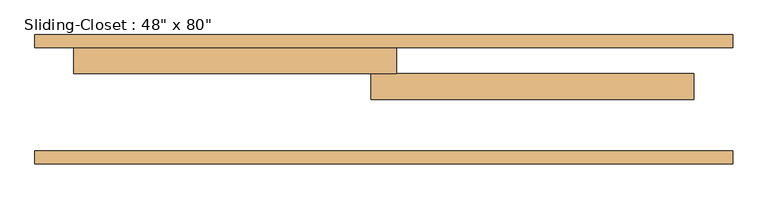
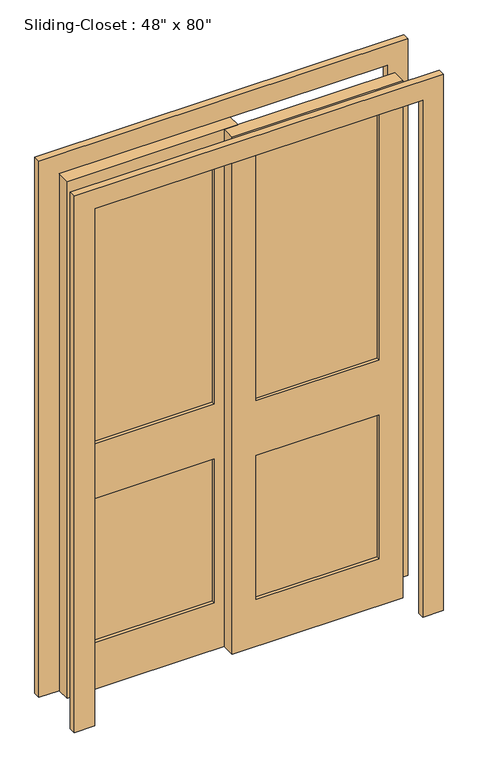
"""IFC4 building model written with IfcOpenShell, lengths in millimetres: door geometry."""

import ifcopenshell
import ifcopenshell.guid

model = None  # the IFC model being written
_history = None  # IfcOwnerHistory: only IFC2X3 demands one
_inside = {}  # id of a spatial element -> (the spatial element, [elements in it])
_under = {}  # id of a project, library or spatial element -> (it, [spatial elements below it])
_declared = {}  # id of a project -> (the project, [libraries it declares])
_typed = {}  # id of a type object -> (the type object, [elements of that type])
_made_of = {}  # id of a material, layer set ... -> (it, [elements and type objects made of it])


def new_model(schema):
    """Start an empty IFC model of exactly this schema.

    Asked for "IFC4X3", IfcOpenShell would pick the latest addendum, in which some entities
    have other attributes; the version numbers below select the first issue.
    IFC2X3 requires an IfcOwnerHistory on every rooted entity: one is made here for all.
    """
    global model, _history
    if schema == "IFC4X3":
        model = ifcopenshell.file(schema_version=(4, 3, 0, 0))
    else:
        model = ifcopenshell.file(schema=schema)
    _inside.clear()
    _under.clear()
    _declared.clear()
    _typed.clear()
    _made_of.clear()
    _history = None
    if model.schema == "IFC2X3":
        org = make("IfcOrganization", Name="unknown")
        user = make(
            "IfcPersonAndOrganization",
            ThePerson=make("IfcPerson", FamilyName="unknown"),
            TheOrganization=org,
        )
        app = make(
            "IfcApplication",
            ApplicationDeveloper=org,
            Version="unknown",
            ApplicationFullName="unknown",
            ApplicationIdentifier="unknown",
        )
        _history = make(
            "IfcOwnerHistory",
            OwningUser=user,
            OwningApplication=app,
            ChangeAction="ADDED",
            CreationDate=0,
        )
    return model


def make(cls, **values):
    """One entity of the class cls with the attributes given. An attribute that is None is left unset."""
    return model.create_entity(
        cls, **{name: value for name, value in values.items() if value is not None}
    )


def rooted(cls, **values):
    """An entity with a GlobalId (a new one), such as an element, a storey or a relation."""
    return make(cls, GlobalId=ifcopenshell.guid.new(), OwnerHistory=_history, **values)


def si_unit(unit_type, name, prefix=None):
    """IfcSIUnit, for example si_unit("LENGTHUNIT", "METRE", prefix="MILLI")."""
    return make("IfcSIUnit", UnitType=unit_type, Prefix=prefix, Name=name)


def assignment(units):
    """IfcUnitAssignment: the units of a project."""
    return None if units is None else make("IfcUnitAssignment", Units=units)


def point(xyz):
    """IfcCartesianPoint."""
    return None if xyz is None else make("IfcCartesianPoint", Coordinates=xyz)


def direction(xyz):
    """IfcDirection."""
    return None if xyz is None else make("IfcDirection", DirectionRatios=xyz)


def frame(location, z_axis=None, x_axis=None):
    """IfcAxis2Placement3D, a coordinate frame: its origin and axes. An axis left out is left unset."""
    return make(
        "IfcAxis2Placement3D",
        Location=point(location),
        Axis=direction(z_axis),
        RefDirection=direction(x_axis),
    )


def origin():
    """The frame at (0, 0, 0) with its axes left unset."""
    return frame((0.0, 0.0, 0.0))


def place(relative_to, where):
    """IfcLocalPlacement: puts the frame where relative to a parent placement (None: the world)."""
    return make(
        "IfcLocalPlacement", PlacementRelTo=relative_to, RelativePlacement=where
    )


def context(
    kind, dimensions, precision=None, world=None, true_north=None, identifier=None
):
    """IfcGeometricRepresentationContext, for example the 3D "Model" context."""
    return make(
        "IfcGeometricRepresentationContext",
        ContextIdentifier=identifier,
        ContextType=kind,
        CoordinateSpaceDimension=dimensions,
        Precision=precision,
        WorldCoordinateSystem=world,
        TrueNorth=true_north,
    )


def project(units=None, contexts=None):
    """IfcProject with its units and contexts."""
    return rooted(
        "IfcProject",
        Name="project",
        RepresentationContexts=contexts,
        UnitsInContext=assignment(units),
    )


def spatial(cls, under=None, at=None, **own):
    """A site, building, storey or space (cls), placed at a placement, below another one or the project."""
    s = rooted(cls, ObjectPlacement=at, **own)
    if under is not None:
        _under.setdefault(under.id(), (under, []))[1].append(s)
    return s


def polyline(points):
    """IfcPolyline through the points."""
    return make("IfcPolyline", Points=[point(p) for p in points])


def outline(outer, holes=None, kind="AREA"):
    """IfcArbitraryClosedProfileDef: a profile drawn as a closed curve; with holes, ...WithVoids."""
    if holes is None:
        return make("IfcArbitraryClosedProfileDef", ProfileType=kind, OuterCurve=outer)
    return make(
        "IfcArbitraryProfileDefWithVoids",
        ProfileType=kind,
        OuterCurve=outer,
        InnerCurves=holes,
    )


def extrude(swept, where, along, depth):
    """IfcExtrudedAreaSolid: the profile swept, set in the frame where, extruded along a direction by depth."""
    return make(
        "IfcExtrudedAreaSolid",
        SweptArea=swept,
        Position=where,
        ExtrudedDirection=direction(along),
        Depth=depth,
    )


def shape(context_of_items, identifier, shape_type, items):
    """IfcShapeRepresentation: the items that make up one representation, for example the "Body"."""
    return make(
        "IfcShapeRepresentation",
        ContextOfItems=context_of_items,
        RepresentationIdentifier=identifier,
        RepresentationType=shape_type,
        Items=items,
    )


def source(mapping_origin, context_of_items, identifier, shape_type, items):
    """IfcRepresentationMap: a shape defined once, which mapped items show again and again."""
    return make(
        "IfcRepresentationMap",
        MappingOrigin=mapping_origin,
        MappedRepresentation=shape(context_of_items, identifier, shape_type, items),
    )


def transform(
    local_origin,
    x_axis=None,
    y_axis=None,
    z_axis=None,
    scale=None,
    scale2=None,
    scale3=None,
    uniform=True,
):
    """IfcCartesianTransformationOperator3D, or its non-uniform kind. x_axis, y_axis, z_axis: its Axis1, 2, 3."""
    if uniform:
        return make(
            "IfcCartesianTransformationOperator3D",
            Axis1=direction(x_axis),
            Axis2=direction(y_axis),
            LocalOrigin=point(local_origin),
            Scale=scale,
            Axis3=direction(z_axis),
        )
    return make(
        "IfcCartesianTransformationOperator3DnonUniform",
        Axis1=direction(x_axis),
        Axis2=direction(y_axis),
        LocalOrigin=point(local_origin),
        Scale=scale,
        Axis3=direction(z_axis),
        Scale2=scale2,
        Scale3=scale3,
    )


def mapped(mapping_source, mapping_target):
    """IfcMappedItem: shows the shape of a source again, moved by a transform."""
    return make(
        "IfcMappedItem", MappingSource=mapping_source, MappingTarget=mapping_target
    )


def made_of(thing, what):
    """Note that an element or type object is made of a material, layer set ...; save() writes the relation."""
    if what is not None:
        _made_of.setdefault(what.id(), (what, []))[1].append(thing)
    return thing


def element(
    cls,
    number,
    at=None,
    inside=None,
    cuts=None,
    type_object=None,
    material=None,
    context=None,
    identifier="Body",
    shape_type=None,
    held_by="IfcProductDefinitionShape",
    body=None,
    shapes=None,
    **own,
):
    """One element of the class cls, such as IfcWall. Its Tag is "e" and its number.

    at: its placement. inside: the storey or other place that contains it. cuts: it is an
    opening in that element (IfcRelVoidsElement). A single representation is given by context,
    identifier, shape_type and body (its items); several are given by shapes. held_by: the class
    of the entity that holds the representations. save() writes the other relations.
    """
    e = rooted(cls, Tag="e%d" % number, ObjectPlacement=at, **own)
    if body is not None:
        shapes = [shape(context, identifier, shape_type, body)]
    if shapes is not None:
        e.Representation = make(held_by, Representations=shapes)
    if inside is not None:
        _inside.setdefault(inside.id(), (inside, []))[1].append(e)
    if cuts is not None:
        rooted(
            "IfcRelVoidsElement", RelatingBuildingElement=cuts, RelatedOpeningElement=e
        )
    if type_object is not None:
        _typed.setdefault(type_object.id(), (type_object, []))[1].append(e)
    return made_of(e, material)


def aggregate(whole, parts):
    """IfcRelAggregates: a whole, such as a stair, and the parts it consists of."""
    return rooted("IfcRelAggregates", RelatingObject=whole, RelatedObjects=parts)


def save(model, path):
    """Write the relations noted so far, then the file.

    IfcRelAggregates (storeys below a building ...), IfcRelContainedInSpatialStructure (elements
    in a storey), IfcRelDefinesByType, IfcRelAssociatesMaterial and IfcRelDeclares: one each for
    every whole, place, type object, material and project.
    """
    for whole, parts in _under.values():
        aggregate(whole, parts)
    for where, things in _inside.values():
        rooted(
            "IfcRelContainedInSpatialStructure",
            RelatedElements=things,
            RelatingStructure=where,
        )
    for kind, things in _typed.values():
        rooted("IfcRelDefinesByType", RelatedObjects=things, RelatingType=kind)
    for what, things in _made_of.values():
        rooted("IfcRelAssociatesMaterial", RelatedObjects=things, RelatingMaterial=what)
    for by, libraries in _declared.values():
        rooted("IfcRelDeclares", RelatingContext=by, RelatedDefinitions=libraries)
    model.write(path)


def door_5d877b8f(model_context):
    return source(origin(), model_context, "Body", "SweptSolid", [
        extrude(outline(polyline([(-63.5, 190.5), (-520.7, 190.5), (-520.7, 215.9), (-63.5, 215.9), (-63.5, 190.5)])), frame((0.0, 0.0, 965.2), z_axis=(0.0, 0.0, 1.0), x_axis=(1.0, 0.0, 0.0)), (0.0, 0.0, 1.0), 977.9),
        extrude(outline(polyline([(-63.5, 190.5), (-520.7, 190.5), (-520.7, 215.9), (-63.5, 215.9), (-63.5, 190.5)])), frame((0.0, 0.0, 184.15), z_axis=(0.0, 0.0, 1.0), x_axis=(1.0, 0.0, 0.0)), (0.0, 0.0, 1.0), 565.15),
        extrude(outline(polyline([(63.5, 165.1), (520.7, 165.1), (520.7, 139.7), (63.5, 139.7), (63.5, 165.1)])), frame((0.0, 0.0, 965.2), z_axis=(0.0, 0.0, 1.0), x_axis=(1.0, 0.0, 0.0)), (0.0, 0.0, 1.0), 977.9),
        extrude(outline(polyline([(63.5, 165.1), (520.7, 165.1), (520.7, 139.7), (63.5, 139.7), (63.5, 165.1)])), frame((0.0, 0.0, 184.15), z_axis=(0.0, 0.0, 1.0), x_axis=(1.0, 0.0, 0.0)), (0.0, 0.0, 1.0), 565.15),
        extrude(outline(polyline([(2032.0, 25.4), (2032.0, -609.6), (0.0, -609.6), (0.0, 25.4), (2032.0, 25.4)]), holes=[polyline([(184.15, -520.7), (749.3, -520.7), (749.3, -63.5), (184.15, -63.5), (184.15, -520.7)]), polyline([(965.2, -520.7), (1943.1, -520.7), (1943.1, -63.5), (965.2, -63.5), (965.2, -520.7)])]), frame((0.0, 177.8, 0.0), z_axis=(0.0, 1.0, 0.0), x_axis=(0.0, 0.0, 1.0)), (0.0, 0.0, 1.0), 50.8),
        extrude(outline(polyline([(0.0, -685.8), (0.0, -609.6), (2032.0, -609.6), (2032.0, 609.6), (0.0, 609.6), (0.0, 685.8), (2108.2, 685.8), (2108.2, -685.8), (0.0, -685.8)])), frame((0.0, 0.0, 0.0), z_axis=(0.0, 1.0, 0.0), x_axis=(0.0, 0.0, 1.0)), (0.0, 0.0, 1.0), 25.4),
        extrude(outline(polyline([(0.0, 685.8), (2108.2, 685.8), (2108.2, -685.8), (0.0, -685.8), (0.0, -609.6), (2032.0, -609.6), (2032.0, 609.6), (0.0, 609.6), (0.0, 685.8)])), frame((0.0, 228.6, 0.0), z_axis=(0.0, 1.0, 0.0), x_axis=(0.0, 0.0, 1.0)), (0.0, 0.0, 1.0), 25.4),
        extrude(outline(polyline([(2032.0, -25.4), (0.0, -25.4), (0.0, 609.6), (2032.0, 609.6), (2032.0, -25.4)]), holes=[polyline([(965.2, 520.7), (965.2, 63.5), (1943.1, 63.5), (1943.1, 520.7), (965.2, 520.7)]), polyline([(184.15, 520.7), (184.15, 63.5), (749.3, 63.5), (749.3, 520.7), (184.15, 520.7)])]), frame((0.0, 127.0, 0.0), z_axis=(0.0, 1.0, 0.0), x_axis=(0.0, 0.0, 1.0)), (0.0, 0.0, 1.0), 50.8),
    ])


if __name__ == "__main__":
    model = new_model("IFC4")
    model_context = context("Model", 3, world=origin())
    ifc_project = project(units=[si_unit("LENGTHUNIT", "METRE", prefix="MILLI")], contexts=[model_context])
    site = spatial("IfcSite", under=ifc_project)
    building = spatial("IfcBuilding", under=site)
    placement = place(None, origin())
    door_shape = door_5d877b8f(model_context)
    element("IfcDoor", 1, ObjectType="Sliding-Closet : 48\" x 80\"", at=placement, inside=building, context=model_context, shape_type="MappedRepresentation", body=[
        mapped(door_shape, transform((0.0, 0.0, 0.0), x_axis=(1.0, 0.0, 0.0), y_axis=(0.0, 1.0, 0.0), z_axis=(0.0, 0.0, 1.0))),
    ])
    save(model, "model.ifc")

# Revit data of these elements
# Type "Sliding-Closet : 48\" x 80\""
#   Type Mark = "54"
#   Assembly Code = "C1020"
#   Thickness = 0' - 2"
#   Height = 6' - 8"
#   Trim Projection Ext = 0' - 1"
#   Trim Projection Int = 0' - 1"
#   Trim Width = 0' - 3"
#   Width = 4' - 0"
#   Define Thermal Properties by = 0
#   Function = 0
#   Door Material = Door - Panel
#   Frame Material = Door - Frame
#   Wall Closure = (empty or 0)
# Element 1 (IfcDoor, "Sliding-Closet : 48\" x 80\"")
#   Materials on its faces: "Door - Panel", "Door - Frame"
# Materials
#   "Door - Panel": class "Wood", colour RGB 227 170 128, transparency 0, Cost = 0
#   "Door - Frame": class "Miscellaneous", colour RGB 153 76 43, transparency 0, Cost = 0
